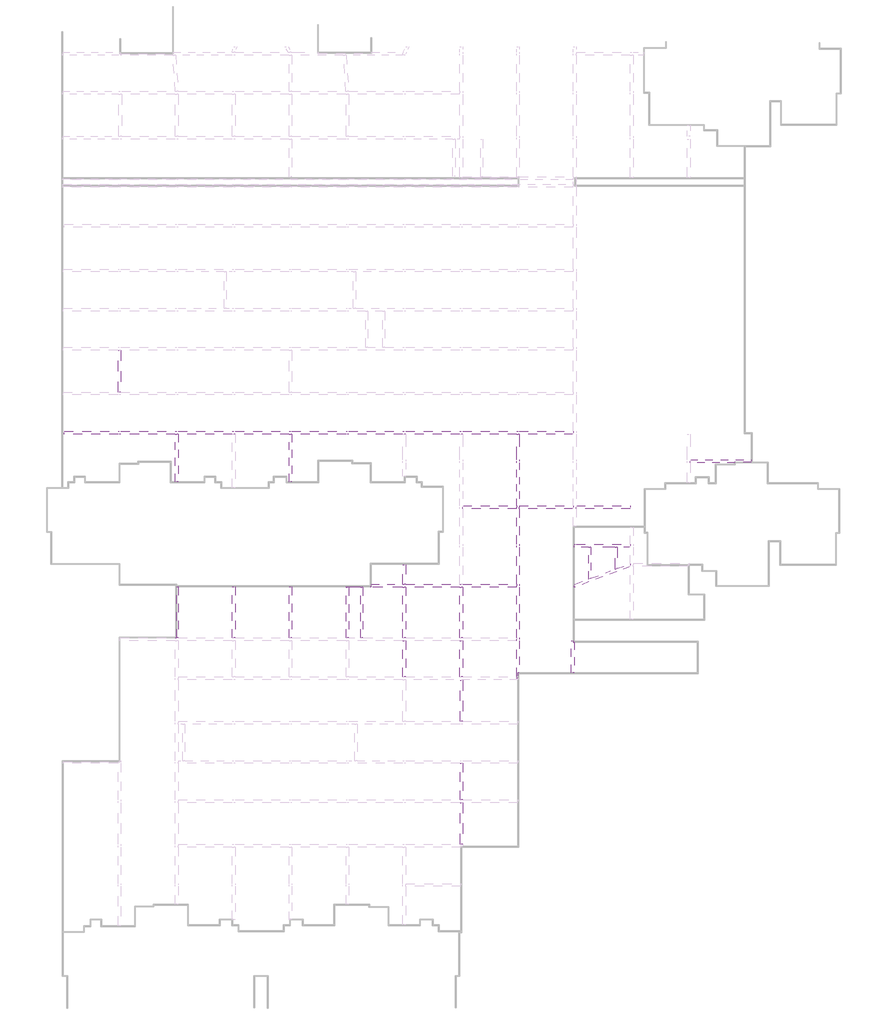
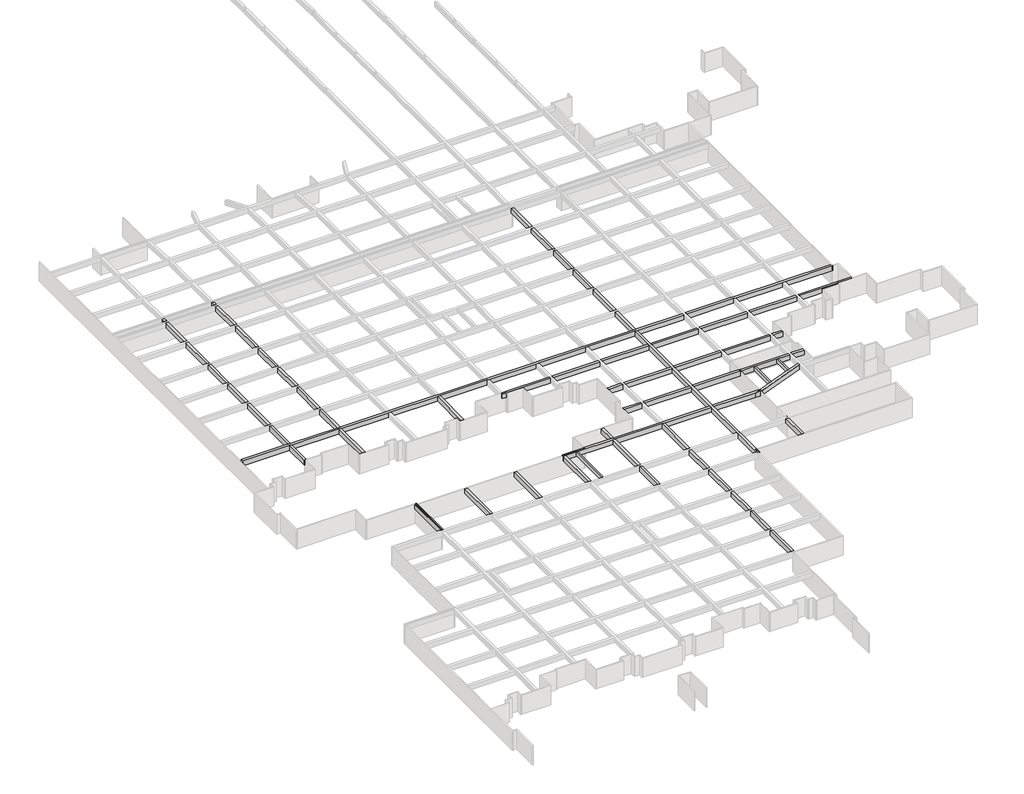
# One storey, part 8 of 14: 28 beams.
"""IFC4 building model written with IfcOpenShell, lengths in millimetres."""

from ifc_helpers import new_model, si_unit, frame, origin, place, context, project, spatial, polyline, outline, extrude, faceted_brep, element, save

model = new_model("IFC4")

# Units and contexts
model_context = context("Model", 3, world=origin())
ifc_project = project(units=[si_unit("LENGTHUNIT", "METRE", prefix="MILLI")], contexts=[model_context])

# Site, building, storey
site = spatial("IfcSite", under=ifc_project)
building = spatial("IfcBuilding", under=site)
storey = spatial("IfcBuildingStorey", under=building, Name="户型图", Elevation=0.0)

# Beams
placement = place(None, origin())
element("IfcBeam", 1, ObjectType="混凝土 - 矩形梁 : KL_beam", at=placement, inside=storey, context=model_context, shape_type="Brep", body=[
    faceted_brep([(-593917.6529954, -163759.4327531, 3300.0), (-593917.6529954, -163759.4327531, 2500.0), (-593917.6529954, -164159.4327531, 2500.0), (-593917.6529954, -164159.4327531, 3300.0), (-522267.6529954, -163759.4327531, 3300.0), (-522267.6529954, -164159.4327531, 3300.0), (-522267.6529954, -164159.4327531, 2500.0), (-522267.6529954, -163759.4327531, 2500.0), (-586331.2602569, -164159.4327531, 3300.0), (-585931.2602569, -164159.4327531, 3300.0), (-578267.6529954, -164159.4327531, 3300.0), (-577867.6529954, -164159.4327531, 3300.0), (-570267.6529954, -164159.4327531, 3300.0), (-569867.6529954, -164159.4327531, 3300.0), (-562267.6529954, -164159.4327531, 3300.0), (-561867.6529954, -164159.4327531, 3300.0), (-554267.6529954, -164159.4327531, 3300.0), (-553867.6529954, -164159.4327531, 3300.0), (-546267.6529954, -164159.4327531, 3300.0), (-545867.6529954, -164159.4327531, 3300.0), (-538267.6529954, -164159.4327531, 3300.0), (-537867.6529954, -164159.4327531, 3300.0), (-530267.6529954, -164159.4327531, 3300.0), (-529867.6529954, -164159.4327531, 3300.0), (-529867.6529954, -163759.4327531, 3300.0), (-530267.6529954, -163759.4327531, 3300.0), (-537867.6529954, -163759.4327531, 3300.0), (-538267.6529954, -163759.4327531, 3300.0), (-545867.6529954, -163759.4327531, 3300.0), (-546267.6529954, -163759.4327531, 3300.0), (-553867.6529954, -163759.4327531, 3300.0), (-554267.6529954, -163759.4327531, 3300.0), (-561867.6529954, -163759.4327531, 3300.0), (-562267.6529954, -163759.4327531, 3300.0), (-569867.6529954, -163759.4327531, 3300.0), (-570267.6529954, -163759.4327531, 3300.0), (-577867.6529954, -163759.4327531, 3300.0), (-578267.6529954, -163759.4327531, 3300.0), (-585931.2602569, -163759.4327531, 3300.0), (-586331.2602569, -163759.4327531, 3300.0), (-586331.2602569, -164159.4327531, 2500.0), (-585931.2602569, -164159.4327531, 2500.0), (-578267.6529954, -164159.4327531, 2500.0), (-577867.6529954, -164159.4327531, 2500.0), (-570267.6529954, -164159.4327531, 2500.0), (-569867.6529954, -164159.4327531, 2500.0), (-562267.6529954, -164159.4327531, 2500.0), (-561867.6529954, -164159.4327531, 2500.0), (-554267.6529954, -164159.4327531, 2500.0), (-553867.6529954, -164159.4327531, 2500.0), (-546267.6529954, -164159.4327531, 2500.0), (-545867.6529954, -164159.4327531, 2500.0), (-538267.6529954, -164159.4327531, 2500.0), (-537867.6529954, -164159.4327531, 2500.0), (-530267.6529954, -164159.4327531, 2500.0), (-529867.6529954, -164159.4327531, 2500.0), (-586331.2602569, -163759.4327531, 2500.0), (-585931.2602569, -163759.4327531, 2500.0), (-578267.6529954, -163759.4327531, 2500.0), (-577867.6529954, -163759.4327531, 2500.0), (-570267.6529954, -163759.4327531, 2500.0), (-569867.6529954, -163759.4327531, 2500.0), (-562267.6529954, -163759.4327531, 2500.0), (-561867.6529954, -163759.4327531, 2500.0), (-554267.6529954, -163759.4327531, 2500.0), (-553867.6529954, -163759.4327531, 2500.0), (-546267.6529954, -163759.4327531, 2500.0), (-545867.6529954, -163759.4327531, 2500.0), (-538267.6529954, -163759.4327531, 2500.0), (-537867.6529954, -163759.4327531, 2500.0), (-530267.6529954, -163759.4327531, 2500.0), (-529867.6529954, -163759.4327531, 2500.0)], [[[0, 1, 2, 3]], [[4, 5, 6, 7]], [[0, 3, 8, 9, 10, 11, 12, 13, 14, 15, 16, 17, 18, 19, 20, 21, 22, 23, 5, 4, 24, 25, 26, 27, 28, 29, 30, 31, 32, 33, 34, 35, 36, 37, 38, 39]], [[3, 2, 40, 41, 42, 43, 44, 45, 46, 47, 48, 49, 50, 51, 52, 53, 54, 55, 6, 5, 23, 22, 21, 20, 19, 18, 17, 16, 15, 14, 13, 12, 11, 10, 9, 8]], [[2, 1, 56, 57, 58, 59, 60, 61, 62, 63, 64, 65, 66, 67, 68, 69, 70, 71, 7, 6, 55, 54, 53, 52, 51, 50, 49, 48, 47, 46, 45, 44, 43, 42, 41, 40]], [[1, 0, 39, 38, 37, 36, 35, 34, 33, 32, 31, 30, 29, 28, 27, 26, 25, 24, 4, 7, 71, 70, 69, 68, 67, 66, 65, 64, 63, 62, 61, 60, 59, 58, 57, 56]]]),
    faceted_brep([(-498227.6529954, -164119.4327531, 3300.0), (-498227.6529954, -163999.4327531, 3300.0), (-498227.6529954, -163759.4327531, 3300.0), (-505867.6529954, -163759.4327531, 3300.0), (-506267.6529954, -163759.4327531, 3300.0), (-513867.6529954, -163759.4327531, 3300.0), (-514267.6529954, -163759.4327531, 3300.0), (-521867.6529954, -163759.4327531, 3300.0), (-521867.6529954, -164159.4327531, 3300.0), (-514267.6529954, -164159.4327531, 3300.0), (-513867.6529954, -164159.4327531, 3300.0), (-506267.6529954, -164159.4327531, 3300.0), (-505867.6529954, -164159.4327531, 3300.0), (-498107.6529954, -164159.4327531, 3300.0), (-498107.6529954, -164119.4327531, 3300.0), (-498107.6529954, -164159.4327531, 2500.0), (-521867.6529954, -164159.4327531, 2500.0), (-514267.6529954, -164159.4327531, 2500.0), (-513867.6529954, -164159.4327531, 2500.0), (-506267.6529954, -164159.4327531, 2500.0), (-505867.6529954, -164159.4327531, 2500.0), (-498227.6529954, -163759.4327531, 2500.0), (-498227.6529954, -164119.4327531, 2500.0), (-498107.6529954, -164119.4327531, 2500.0), (-521867.6529954, -163759.4327531, 2500.0), (-514267.6529954, -163759.4327531, 2500.0), (-513867.6529954, -163759.4327531, 2500.0), (-506267.6529954, -163759.4327531, 2500.0), (-505867.6529954, -163759.4327531, 2500.0)], [[[0, 1, 2, 3, 4, 5, 6, 7, 8, 9, 10, 11, 12, 13, 14]], [[15, 13, 12, 11, 10, 9, 8, 16, 17, 18, 19, 20]], [[21, 22, 23, 15, 20, 19, 18, 17, 16, 24, 25, 26, 27, 28]], [[2, 21, 28, 27, 26, 25, 24, 7, 6, 5, 4, 3]], [[13, 15, 23, 14]], [[0, 22, 21, 2, 1]], [[8, 7, 24, 16]], [[22, 0, 14, 23]]]),
])
element("IfcBeam", 2, ObjectType="混凝土 - 矩形梁 : KL_beam", at=placement, inside=storey, context=model_context, shape_type="Brep", body=[
    faceted_brep([(-586191.2602569, -168257.8565288, 3300.0), (-586071.2602569, -168257.8565288, 3300.0), (-585931.2602569, -168257.8565288, 3300.0), (-585931.2602569, -164159.4327531, 3300.0), (-586331.2602569, -164159.4327531, 3300.0), (-586331.2602569, -168377.8565288, 3300.0), (-586191.2602569, -168377.8565288, 3300.0), (-585931.2602569, -168257.8565288, 2500.0), (-585931.2602569, -164159.4327531, 2500.0), (-586191.2602569, -168257.8565288, 2500.0), (-586191.2602569, -168377.8565288, 2500.0), (-586331.2602569, -168377.8565288, 2500.0), (-586331.2602569, -164159.4327531, 2500.0)], [[[0, 1, 2, 3, 4, 5, 6]], [[2, 7, 8, 3]], [[7, 9, 10, 11, 12, 8]], [[11, 5, 4, 12]], [[5, 11, 10, 6]], [[0, 9, 7, 2, 1]], [[4, 3, 8, 12]], [[9, 0, 6, 10]]]),
    faceted_brep([(-586331.2602569, -128359.4327532, 3300.0), (-585931.2602569, -128359.4327532, 3300.0), (-585931.2602569, -128359.4327532, 2500.0), (-586331.2602569, -128359.4327532, 2500.0), (-585931.2602569, -129034.4327531, 3300.0), (-586331.2602569, -129034.4327531, 3300.0), (-586331.2602569, -129034.4327531, 2500.0), (-585931.2602569, -129034.4327531, 2500.0)], [[[0, 1, 2, 3]], [[4, 5, 6, 7]], [[1, 0, 5, 4]], [[2, 1, 4, 7]], [[3, 2, 7, 6]], [[0, 3, 6, 5]]]),
    faceted_brep([(-586331.2602569, -129434.4327531, 3300.0), (-585931.2602569, -129434.4327531, 3300.0), (-585931.2602569, -129434.4327531, 2500.0), (-586331.2602569, -129434.4327531, 2500.0), (-585931.2602569, -134659.4327531, 3300.0), (-586331.2602569, -134659.4327531, 3300.0), (-586331.2602569, -134659.4327531, 2500.0), (-585931.2602569, -134659.4327531, 2500.0)], [[[0, 1, 2, 3]], [[4, 5, 6, 7]], [[1, 0, 5, 4]], [[2, 1, 4, 7]], [[3, 2, 7, 6]], [[0, 3, 6, 5]]]),
    faceted_brep([(-586331.2602569, -135059.4327531, 3300.0), (-585931.2602569, -135059.4327531, 3300.0), (-585931.2602569, -135059.4327531, 2500.0), (-586331.2602569, -135059.4327531, 2500.0), (-585931.2602569, -140959.4327531, 3300.0), (-586331.2602569, -140959.4327531, 3300.0), (-586331.2602569, -140959.4327531, 2500.0), (-585931.2602569, -140959.4327531, 2500.0)], [[[0, 1, 2, 3]], [[4, 5, 6, 7]], [[1, 0, 5, 4]], [[2, 1, 4, 7]], [[3, 2, 7, 6]], [[0, 3, 6, 5]]]),
    faceted_brep([(-586331.2602569, -141359.4327531, 3300.0), (-585931.2602569, -141359.4327531, 3300.0), (-585931.2602569, -141359.4327531, 2500.0), (-586331.2602569, -141359.4327531, 2500.0), (-585931.2602569, -146459.4327531, 3300.0), (-586331.2602569, -146459.4327531, 3300.0), (-586331.2602569, -146459.4327531, 2500.0), (-585931.2602569, -146459.4327531, 2500.0)], [[[0, 1, 2, 3]], [[4, 5, 6, 7]], [[1, 0, 5, 4]], [[2, 1, 4, 7]], [[3, 2, 7, 6]], [[0, 3, 6, 5]]]),
    faceted_brep([(-586331.2602569, -146859.4327531, 3300.0), (-585931.2602569, -146859.4327531, 3300.0), (-585931.2602569, -146859.4327531, 2500.0), (-586331.2602569, -146859.4327531, 2500.0), (-585931.2602569, -151959.4327531, 3300.0), (-586331.2602569, -151959.4327531, 3300.0), (-586331.2602569, -151959.4327531, 2500.0), (-585931.2602569, -151959.4327531, 2500.0)], [[[0, 1, 2, 3]], [[4, 5, 6, 7]], [[1, 0, 5, 4]], [[2, 1, 4, 7]], [[3, 2, 7, 6]], [[0, 3, 6, 5]]]),
    faceted_brep([(-586331.2602569, -152359.4327531, 3300.0), (-585931.2602569, -152359.4327531, 3300.0), (-585931.2602569, -152359.4327531, 2500.0), (-586331.2602569, -152359.4327531, 2500.0), (-585931.2602569, -158259.4327531, 3300.0), (-586331.2602569, -158259.4327531, 3300.0), (-586331.2602569, -158259.4327531, 2500.0), (-585931.2602569, -158259.4327531, 2500.0)], [[[0, 1, 2, 3]], [[4, 5, 6, 7]], [[1, 0, 5, 4]], [[2, 1, 4, 7]], [[3, 2, 7, 6]], [[0, 3, 6, 5]]]),
    faceted_brep([(-586331.2602569, -158659.4327531, 3300.0), (-585931.2602569, -158659.4327531, 3300.0), (-585931.2602569, -158659.4327531, 2500.0), (-586331.2602569, -158659.4327531, 2500.0), (-585931.2602569, -163759.4327531, 3300.0), (-586331.2602569, -163759.4327531, 3300.0), (-586331.2602569, -163759.4327531, 2500.0), (-585931.2602569, -163759.4327531, 2500.0)], [[[0, 1, 2, 3]], [[4, 5, 6, 7]], [[1, 0, 5, 4]], [[2, 1, 4, 7]], [[3, 2, 7, 6]], [[0, 3, 6, 5]]]),
])
element("IfcBeam", 3, ObjectType="混凝土 - 矩形梁 : KL_beam", at=placement, inside=storey, context=model_context, shape_type="SweptSolid", body=[
    extrude(outline(polyline([(-578267.6529954, -128359.4327532), (-577867.6529954, -128359.4327532), (-577867.6529954, -129034.4327531), (-578267.6529954, -129034.4327531), (-578267.6529954, -128359.4327532)])), frame((0.0, 0.0, 2500.0), z_axis=(0.0, 0.0, 1.0), x_axis=(1.0, 0.0, 0.0)), (0.0, 0.0, 1.0), 800.0),
    extrude(outline(polyline([(-577867.6529954, -170882.8565379), (-578267.6529954, -170882.8565379), (-578267.6529954, -164159.4327531), (-577867.6529954, -164159.4327531), (-577867.6529954, -170882.8565379)])), frame((0.0, 0.0, 2500.0), z_axis=(0.0, 0.0, 1.0), x_axis=(1.0, 0.0, 0.0)), (0.0, 0.0, 1.0), 800.0),
    extrude(outline(polyline([(-578267.6529954, -129434.4327531), (-577867.6529954, -129434.4327531), (-577867.6529954, -134659.4327531), (-578267.6529954, -134659.4327531), (-578267.6529954, -129434.4327531)])), frame((0.0, 0.0, 2500.0), z_axis=(0.0, 0.0, 1.0), x_axis=(1.0, 0.0, 0.0)), (0.0, 0.0, 1.0), 800.0),
    extrude(outline(polyline([(-578267.6529954, -135059.4327531), (-577867.6529954, -135059.4327531), (-577867.6529954, -140959.4327531), (-578267.6529954, -140959.4327531), (-578267.6529954, -135059.4327531)])), frame((0.0, 0.0, 2500.0), z_axis=(0.0, 0.0, 1.0), x_axis=(1.0, 0.0, 0.0)), (0.0, 0.0, 1.0), 800.0),
    extrude(outline(polyline([(-578267.6529954, -141359.4327531), (-577867.6529954, -141359.4327531), (-577867.6529954, -146459.4327531), (-578267.6529954, -146459.4327531), (-578267.6529954, -141359.4327531)])), frame((0.0, 0.0, 2500.0), z_axis=(0.0, 0.0, 1.0), x_axis=(1.0, 0.0, 0.0)), (0.0, 0.0, 1.0), 800.0),
    extrude(outline(polyline([(-578267.6529954, -146859.4327531), (-577867.6529954, -146859.4327531), (-577867.6529954, -151959.4327531), (-578267.6529954, -151959.4327531), (-578267.6529954, -146859.4327531)])), frame((0.0, 0.0, 2500.0), z_axis=(0.0, 0.0, 1.0), x_axis=(1.0, 0.0, 0.0)), (0.0, 0.0, 1.0), 800.0),
    extrude(outline(polyline([(-578267.6529954, -152359.4327531), (-577867.6529954, -152359.4327531), (-577867.6529954, -158259.4327531), (-578267.6529954, -158259.4327531), (-578267.6529954, -152359.4327531)])), frame((0.0, 0.0, 2500.0), z_axis=(0.0, 0.0, 1.0), x_axis=(1.0, 0.0, 0.0)), (0.0, 0.0, 1.0), 800.0),
    extrude(outline(polyline([(-578267.6529954, -158659.4327531), (-577867.6529954, -158659.4327531), (-577867.6529954, -163759.4327531), (-578267.6529954, -163759.4327531), (-578267.6529954, -158659.4327531)])), frame((0.0, 0.0, 2500.0), z_axis=(0.0, 0.0, 1.0), x_axis=(1.0, 0.0, 0.0)), (0.0, 0.0, 1.0), 800.0),
])
element("IfcBeam", 4, ObjectType="混凝土 - 矩形梁 : KL_beam", at=placement, inside=storey, context=model_context, shape_type="Brep", body=[
    faceted_brep([(-529867.6529954, -198534.4327531, 2500.0), (-529867.6529954, -198534.4327531, 3300.0), (-529997.7352575, -198534.4327531, 3300.0), (-529997.7352575, -198534.4327531, 2500.0), (-529867.6529954, -197850.9174567, 3300.0), (-529997.7352575, -197850.9174567, 3300.0), (-529867.6529954, -197850.9174567, 2500.0), (-529997.7352575, -197850.9174567, 2500.0)], [[[0, 1, 2, 3]], [[2, 1, 4, 5]], [[1, 0, 6, 4]], [[3, 2, 5, 7]], [[5, 4, 6, 7]], [[0, 3, 7, 6]]]),
    faceted_brep([(-530267.6529954, -198534.4327531, 2500.0), (-530267.6529954, -198534.4327531, 3300.0), (-530267.6529954, -198334.4327531, 3300.0), (-530267.6529954, -193242.8565135, 3300.0), (-530267.6529954, -192842.8565135, 3300.0), (-530267.6529954, -185692.8565135, 3300.0), (-530267.6529954, -185292.8565135, 3300.0), (-530267.6529954, -180052.8565433, 3300.0), (-530267.6529954, -179652.8565433, 3300.0), (-530267.6529954, -174657.5200046, 3300.0), (-530267.6529954, -174257.5200046, 3300.0), (-530267.6529954, -168200.507479, 3300.0), (-530267.6529954, -167800.507479, 3300.0), (-530267.6529954, -164159.4327531, 3300.0), (-530267.6529954, -164159.4327531, 2500.0), (-530267.6529954, -167800.507479, 2500.0), (-530267.6529954, -168200.507479, 2500.0), (-530267.6529954, -174257.5200046, 2500.0), (-530267.6529954, -174657.5200046, 2500.0), (-530267.6529954, -179652.8565433, 2500.0), (-530267.6529954, -180052.8565433, 2500.0), (-530267.6529954, -185292.8565135, 2500.0), (-530267.6529954, -185692.8565135, 2500.0), (-530267.6529954, -192842.8565135, 2500.0), (-530267.6529954, -193242.8565135, 2500.0), (-530267.6529954, -198334.4327531, 2500.0), (-529867.6529954, -164159.4327531, 2500.0), (-529867.6529954, -167800.507479, 2500.0), (-529867.6529954, -168200.507479, 2500.0), (-529867.6529954, -174257.5200046, 2500.0), (-529867.6529954, -174657.5200046, 2500.0), (-529867.6529954, -179652.8565433, 2500.0), (-529867.6529954, -180052.8565433, 2500.0), (-529867.6529954, -185292.8565135, 2500.0), (-529867.6529954, -185692.8565135, 2500.0), (-529867.6529954, -192842.8565135, 2500.0), (-529867.6529954, -193242.8565135, 2500.0), (-529867.6529954, -197730.9174567, 2500.0), (-530117.7352575, -197730.9174567, 2500.0), (-530117.7352575, -198534.4327531, 2500.0), (-529867.6529954, -164159.4327531, 3300.0), (-530117.7352575, -197730.9174567, 3300.0), (-530117.7352575, -198534.4327531, 3300.0), (-529867.6529954, -197730.9174567, 3300.0), (-529997.7352575, -197730.9174567, 3300.0), (-529867.6529954, -193242.8565135, 3300.0), (-529867.6529954, -192842.8565135, 3300.0), (-529867.6529954, -185692.8565135, 3300.0), (-529867.6529954, -185292.8565135, 3300.0), (-529867.6529954, -180052.8565433, 3300.0), (-529867.6529954, -179652.8565433, 3300.0), (-529867.6529954, -174657.5200046, 3300.0), (-529867.6529954, -174257.5200046, 3300.0), (-529867.6529954, -168200.507479, 3300.0), (-529867.6529954, -167800.507479, 3300.0)], [[[0, 1, 2, 3, 4, 5, 6, 7, 8, 9, 10, 11, 12, 13, 14, 15, 16, 17, 18, 19, 20, 21, 22, 23, 24, 25]], [[0, 25, 24, 23, 22, 21, 20, 19, 18, 17, 16, 15, 14, 26, 27, 28, 29, 30, 31, 32, 33, 34, 35, 36, 37, 38, 39]], [[13, 40, 26, 14]], [[38, 41, 42, 39]], [[41, 38, 37, 43, 44]], [[1, 0, 39, 42]], [[13, 12, 11, 10, 9, 8, 7, 6, 5, 4, 3, 2, 1, 42, 41, 44, 43, 45, 46, 47, 48, 49, 50, 51, 52, 53, 54, 40]], [[26, 40, 54, 53, 52, 51, 50, 49, 48, 47, 46, 45, 43, 37, 36, 35, 34, 33, 32, 31, 30, 29, 28, 27]]]),
    faceted_brep([(-530267.6529954, -129434.4327531, 3300.0), (-529867.6529954, -129434.4327531, 3300.0), (-529867.6529954, -129434.4327531, 2500.0), (-530267.6529954, -129434.4327531, 2500.0), (-529867.6529954, -134659.4327531, 3300.0), (-530267.6529954, -134659.4327531, 3300.0), (-530267.6529954, -134659.4327531, 2500.0), (-529867.6529954, -134659.4327531, 2500.0)], [[[0, 1, 2, 3]], [[4, 5, 6, 7]], [[1, 0, 5, 4]], [[0, 3, 6, 5]], [[3, 2, 7, 6]], [[2, 1, 4, 7]]]),
    faceted_brep([(-530267.6529954, -135059.4327531, 3300.0), (-529867.6529954, -135059.4327531, 3300.0), (-529867.6529954, -135059.4327531, 2500.0), (-530267.6529954, -135059.4327531, 2500.0), (-529867.6529954, -140959.4327531, 3300.0), (-530267.6529954, -140959.4327531, 3300.0), (-530267.6529954, -140959.4327531, 2500.0), (-529867.6529954, -140959.4327531, 2500.0)], [[[0, 1, 2, 3]], [[4, 5, 6, 7]], [[1, 0, 5, 4]], [[0, 3, 6, 5]], [[3, 2, 7, 6]], [[2, 1, 4, 7]]]),
    faceted_brep([(-530267.6529954, -141359.4327531, 3300.0), (-529867.6529954, -141359.4327531, 3300.0), (-529867.6529954, -141359.4327531, 2500.0), (-530267.6529954, -141359.4327531, 2500.0), (-529867.6529954, -146459.4327531, 3300.0), (-530267.6529954, -146459.4327531, 3300.0), (-530267.6529954, -146459.4327531, 2500.0), (-529867.6529954, -146459.4327531, 2500.0)], [[[0, 1, 2, 3]], [[4, 5, 6, 7]], [[1, 0, 5, 4]], [[0, 3, 6, 5]], [[3, 2, 7, 6]], [[2, 1, 4, 7]]]),
    faceted_brep([(-530267.6529954, -146859.4327531, 3300.0), (-529867.6529954, -146859.4327531, 3300.0), (-529867.6529954, -146859.4327531, 2500.0), (-530267.6529954, -146859.4327531, 2500.0), (-529867.6529954, -151959.4327531, 3300.0), (-530267.6529954, -151959.4327531, 3300.0), (-530267.6529954, -151959.4327531, 2500.0), (-529867.6529954, -151959.4327531, 2500.0)], [[[0, 1, 2, 3]], [[4, 5, 6, 7]], [[1, 0, 5, 4]], [[0, 3, 6, 5]], [[3, 2, 7, 6]], [[2, 1, 4, 7]]]),
    faceted_brep([(-530267.6529954, -152359.4327531, 3300.0), (-529867.6529954, -152359.4327531, 3300.0), (-529867.6529954, -152359.4327531, 2500.0), (-530267.6529954, -152359.4327531, 2500.0), (-529867.6529954, -158259.4327531, 3300.0), (-530267.6529954, -158259.4327531, 3300.0), (-530267.6529954, -158259.4327531, 2500.0), (-529867.6529954, -158259.4327531, 2500.0)], [[[0, 1, 2, 3]], [[4, 5, 6, 7]], [[1, 0, 5, 4]], [[0, 3, 6, 5]], [[3, 2, 7, 6]], [[2, 1, 4, 7]]]),
    faceted_brep([(-530267.6529954, -158659.4327531, 3300.0), (-529867.6529954, -158659.4327531, 3300.0), (-529867.6529954, -158659.4327531, 2500.0), (-530267.6529954, -158659.4327531, 2500.0), (-529867.6529954, -163759.4327531, 3300.0), (-530267.6529954, -163759.4327531, 3300.0), (-530267.6529954, -163759.4327531, 2500.0), (-529867.6529954, -163759.4327531, 2500.0)], [[[0, 1, 2, 3]], [[4, 5, 6, 7]], [[1, 0, 5, 4]], [[0, 3, 6, 5]], [[3, 2, 7, 6]], [[2, 1, 4, 7]]]),
])
element("IfcBeam", 5, ObjectType="混凝土 - 矩形梁 : KL_beam", at=placement, inside=storey, context=model_context, shape_type="Brep", body=[
    faceted_brep([(-554067.6529954, -168200.507479, 2500.0), (-554067.6529954, -168200.507479, 3300.0), (-554067.6529954, -167952.8565288, 3300.0), (-554067.6529954, -167952.8565288, 2500.0), (-553441.260255, -168200.507479, 3300.0), (-553441.260255, -167952.8565288, 3300.0), (-553441.260255, -168200.507479, 2500.0), (-553441.260255, -167952.8565288, 2500.0)], [[[0, 1, 2, 3]], [[2, 1, 4, 5]], [[1, 0, 6, 4]], [[3, 2, 5, 7]], [[5, 4, 6, 7]], [[0, 3, 7, 6]]]),
    faceted_brep([(-522267.6529954, -167800.507479, 3300.0), (-522267.6529954, -167800.507479, 2500.0), (-529867.6529954, -167800.507479, 2500.0), (-529867.6529954, -167800.507479, 3300.0), (-522267.6529954, -168200.507479, 2500.0), (-529867.6529954, -168200.507479, 2500.0), (-522267.6529954, -168200.507479, 3300.0), (-529867.6529954, -168200.507479, 3300.0)], [[[0, 1, 2, 3]], [[1, 4, 5, 2]], [[0, 6, 4, 1]], [[3, 2, 5, 7]], [[6, 0, 3, 7]], [[4, 6, 7, 5]]]),
    faceted_brep([(-497277.6529954, -167800.507479, 3300.0), (-497277.6529954, -168097.2169847, 3300.0), (-497277.6529954, -168097.2169847, 2500.0), (-497277.6529954, -167800.507479, 2500.0), (-505867.6529954, -168200.507479, 3300.0), (-505867.6529954, -167800.507479, 3300.0), (-505867.6529954, -167800.507479, 2500.0), (-505867.6529954, -168200.507479, 2500.0), (-499624.2878989, -168200.507479, 3300.0), (-499624.2878989, -168097.2169847, 3300.0), (-499504.2878989, -168097.2169847, 3300.0), (-499624.2878989, -168097.2169847, 2500.0), (-499624.2878989, -168200.507479, 2500.0)], [[[0, 1, 2, 3]], [[4, 5, 6, 7]], [[1, 0, 5, 4, 8, 9, 10]], [[0, 3, 6, 5]], [[3, 2, 11, 12, 7, 6]], [[4, 7, 12, 8]], [[2, 1, 10, 9, 11]], [[11, 9, 8, 12]]]),
    faceted_brep([(-521867.6529954, -168200.507479, 3300.0), (-521867.6529954, -167800.507479, 3300.0), (-521867.6529954, -167800.507479, 2500.0), (-521867.6529954, -168200.507479, 2500.0), (-514267.6529954, -168200.507479, 3300.0), (-514267.6529954, -167800.507479, 3300.0), (-514267.6529954, -167800.507479, 2500.0), (-514267.6529954, -168200.507479, 2500.0)], [[[0, 1, 2, 3]], [[1, 0, 4, 5]], [[2, 1, 5, 6]], [[3, 2, 6, 7]], [[0, 3, 7, 4]], [[5, 4, 7, 6]]]),
    faceted_brep([(-553867.6529954, -167800.507479, 3300.0), (-553867.6529954, -167800.507479, 2500.0), (-553867.6529954, -167832.8565288, 2500.0), (-553867.6529954, -167832.8565288, 3300.0), (-546267.6529954, -167800.507479, 3300.0), (-546267.6529954, -168200.507479, 3300.0), (-546267.6529954, -168200.507479, 2500.0), (-546267.6529954, -167800.507479, 2500.0), (-553321.260255, -168200.507479, 2500.0), (-553321.260255, -167832.8565288, 2500.0), (-553321.260255, -167832.8565288, 3300.0), (-553321.260255, -168200.507479, 3300.0), (-553321.260255, -167952.8565288, 3300.0)], [[[0, 1, 2, 3]], [[4, 5, 6, 7]], [[1, 0, 4, 7]], [[1, 7, 6, 8, 9, 2]], [[9, 10, 3, 2]], [[10, 9, 8, 11, 12]], [[4, 0, 3, 10, 12, 11, 5]], [[6, 5, 11, 8]]]),
    faceted_brep([(-545867.6529954, -168200.507479, 3300.0), (-545867.6529954, -167800.507479, 3300.0), (-545867.6529954, -167800.507479, 2500.0), (-545867.6529954, -168200.507479, 2500.0), (-538267.6529954, -168200.507479, 3300.0), (-538267.6529954, -167800.507479, 3300.0), (-538267.6529954, -168200.507479, 2500.0), (-538267.6529954, -167800.507479, 2500.0)], [[[0, 1, 2, 3]], [[1, 0, 4, 5]], [[0, 3, 6, 4]], [[7, 5, 4, 6]], [[2, 1, 5, 7]], [[3, 2, 7, 6]]]),
    faceted_brep([(-537867.6529954, -167800.507479, 3300.0), (-537867.6529954, -167800.507479, 2500.0), (-537867.6529954, -168200.507479, 2500.0), (-537867.6529954, -168200.507479, 3300.0), (-530267.6529954, -168200.507479, 3300.0), (-530267.6529954, -167800.507479, 3300.0), (-530267.6529954, -168200.507479, 2500.0), (-530267.6529954, -167800.507479, 2500.0)], [[[0, 1, 2, 3]], [[0, 3, 4, 5]], [[3, 2, 6, 4]], [[7, 5, 4, 6]], [[1, 0, 5, 7]], [[2, 1, 7, 6]]]),
    faceted_brep([(-513867.6529954, -168200.507479, 3300.0), (-513867.6529954, -167800.507479, 3300.0), (-513867.6529954, -167800.507479, 2500.0), (-513867.6529954, -168200.507479, 2500.0), (-506267.6529954, -168200.507479, 3300.0), (-506267.6529954, -167800.507479, 3300.0), (-506267.6529954, -167800.507479, 2500.0), (-506267.6529954, -168200.507479, 2500.0)], [[[0, 1, 2, 3]], [[1, 0, 4, 5]], [[2, 1, 5, 6]], [[3, 2, 6, 7]], [[0, 3, 7, 4]], [[5, 4, 7, 6]]]),
])
element("IfcBeam", 6, ObjectType="混凝土 - 矩形梁 : KL_beam", at=placement, inside=storey, context=model_context, shape_type="SweptSolid", body=[
    extrude(outline(polyline([(-561867.6529954, -170882.8565379), (-562267.6529954, -170882.8565379), (-562267.6529954, -164159.4327531), (-561867.6529954, -164159.4327531), (-561867.6529954, -170882.8565379)])), frame((0.0, 0.0, 2500.0), z_axis=(0.0, 0.0, 1.0), x_axis=(1.0, 0.0, 0.0)), (0.0, 0.0, 1.0), 800.0),
])
element("IfcBeam", 7, ObjectType="混凝土 - 矩形梁 : KL_beam", at=placement, inside=storey, context=model_context, shape_type="SweptSolid", body=[
    extrude(outline(polyline([(-522267.6529954, -174257.5200046), (-522267.6529954, -174657.5200046), (-529867.6529954, -174657.5200046), (-529867.6529954, -174257.5200046), (-522267.6529954, -174257.5200046)])), frame((0.0, 0.0, 2500.0), z_axis=(0.0, 0.0, 1.0), x_axis=(1.0, 0.0, 0.0)), (0.0, 0.0, 1.0), 800.0),
])
element("IfcBeam", 8, ObjectType="混凝土 - 矩形梁 : KL_beam", at=placement, inside=storey, context=model_context, shape_type="SweptSolid", body=[
    extrude(outline(polyline([(-521867.6529954, -174657.5200046), (-521867.6529954, -174257.5200046), (-514267.6529954, -174257.5200046), (-514267.6529954, -174657.5200046), (-521867.6529954, -174657.5200046)])), frame((0.0, 0.0, 2500.0), z_axis=(0.0, 0.0, 1.0), x_axis=(1.0, 0.0, 0.0)), (0.0, 0.0, 1.0), 800.0),
    extrude(outline(polyline([(-512303.9222774, -174257.5200046), (-512303.9222774, -174657.5200046), (-513867.6529954, -174657.5200046), (-513867.6529954, -174257.5200046), (-512303.9222774, -174257.5200046)])), frame((0.0, 0.0, 2500.0), z_axis=(0.0, 0.0, 1.0), x_axis=(1.0, 0.0, 0.0)), (0.0, 0.0, 1.0), 800.0),
])
element("IfcBeam", 9, ObjectType="混凝土 - 矩形梁 : KL_beam", at=placement, inside=storey, context=model_context, shape_type="SweptSolid", body=[
    extrude(outline(polyline([(-530267.6529954, -174257.5200046), (-530267.6529954, -174657.5200046), (-537867.6529954, -174657.5200046), (-537867.6529954, -174257.5200046), (-530267.6529954, -174257.5200046)])), frame((0.0, 0.0, 2500.0), z_axis=(0.0, 0.0, 1.0), x_axis=(1.0, 0.0, 0.0)), (0.0, 0.0, 1.0), 800.0),
    extrude(outline(polyline([(-540571.2602521, -174657.5200046), (-540571.2602521, -174257.5200046), (-538267.6529954, -174257.5200046), (-538267.6529954, -174657.5200046), (-540571.2602521, -174657.5200046)])), frame((0.0, 0.0, 2500.0), z_axis=(0.0, 0.0, 1.0), x_axis=(1.0, 0.0, 0.0)), (0.0, 0.0, 1.0), 800.0),
])
element("IfcBeam", 10, ObjectType="混凝土 - 矩形梁 : KL_beam", at=placement, inside=storey, context=model_context, shape_type="Brep", body=[
    faceted_brep([(-511864.0912647, -179652.8565433, 3300.0), (-511864.0912647, -180052.8565433, 3300.0), (-511864.0912647, -180052.8565433, 2500.0), (-511864.0912647, -179652.8565433, 2500.0), (-513867.6529954, -179652.8565433, 3300.0), (-513867.6529954, -180052.8565433, 3300.0), (-513867.6529954, -180052.8565433, 2500.0), (-513867.6529954, -179652.8565433, 2500.0)], [[[0, 1, 2, 3]], [[1, 0, 4, 5]], [[2, 1, 5, 6]], [[3, 2, 6, 7]], [[0, 3, 7, 4]], [[5, 4, 7, 6]]]),
    faceted_brep([(-541171.2602521, -180052.8565433, 3300.0), (-541171.2602521, -179652.8565433, 3300.0), (-541171.2602521, -179652.8565433, 2500.0), (-541171.2602521, -180052.8565433, 2500.0), (-538267.6529954, -179652.8565433, 3300.0), (-538267.6529954, -180052.8565433, 3300.0), (-538267.6529954, -180052.8565433, 2500.0), (-538267.6529954, -179652.8565433, 2500.0)], [[[0, 1, 2, 3]], [[4, 5, 6, 7]], [[1, 0, 5, 4]], [[0, 3, 6, 5]], [[3, 2, 7, 6]], [[2, 1, 4, 7]]]),
    faceted_brep([(-537867.6529954, -180052.8565433, 3300.0), (-537867.6529954, -179652.8565433, 3300.0), (-537867.6529954, -179652.8565433, 2500.0), (-537867.6529954, -180052.8565433, 2500.0), (-530267.6529954, -179652.8565433, 3300.0), (-530267.6529954, -180052.8565433, 3300.0), (-530267.6529954, -180052.8565433, 2500.0), (-530267.6529954, -179652.8565433, 2500.0)], [[[0, 1, 2, 3]], [[4, 5, 6, 7]], [[1, 0, 5, 4]], [[0, 3, 6, 5]], [[3, 2, 7, 6]], [[2, 1, 4, 7]]]),
    faceted_brep([(-529867.6529954, -180052.8565433, 3300.0), (-529867.6529954, -179652.8565433, 3300.0), (-529867.6529954, -179652.8565433, 2500.0), (-529867.6529954, -180052.8565433, 2500.0), (-522303.9222774, -179652.8565433, 3300.0), (-522303.9222774, -180052.8565433, 3300.0), (-522303.9222774, -180052.8565433, 2500.0), (-522303.9222774, -179652.8565433, 2500.0)], [[[0, 1, 2, 3]], [[4, 5, 6, 7]], [[1, 0, 5, 4]], [[0, 3, 6, 5]], [[3, 2, 7, 6]], [[2, 1, 4, 7]]]),
    faceted_brep([(-514267.6529954, -179652.8565433, 3300.0), (-514267.6529954, -180052.8565433, 3300.0), (-514267.6529954, -180052.8565433, 2500.0), (-514267.6529954, -179652.8565433, 2500.0), (-521867.6529954, -179652.8565433, 3300.0), (-522183.9222774, -179652.8565433, 3300.0), (-522183.9222774, -180052.8565433, 3300.0), (-520117.6529954, -180052.8565433, 3300.0), (-519817.6529954, -180052.8565433, 3300.0), (-516417.6683344, -180052.8565433, 3300.0), (-516117.6683344, -180052.8565433, 3300.0), (-522183.9222774, -180052.8565433, 2500.0), (-522183.9222774, -179652.8565433, 2500.0), (-521867.6529954, -179652.8565433, 2500.0)], [[[0, 1, 2, 3]], [[1, 0, 4, 5, 6, 7, 8, 9, 10]], [[2, 1, 10, 9, 8, 7, 6, 11]], [[3, 2, 11, 12, 13]], [[0, 3, 13, 12, 5, 4]], [[6, 5, 12, 11]]]),
])
element("IfcBeam", 11, ObjectType="混凝土 - 矩形梁 : KL_beam", at=placement, inside=storey, context=model_context, shape_type="Brep", body=[
    faceted_brep([(-523181.5016488, -185692.8565135, 3300.0), (-522303.9222774, -185692.8565135, 3300.0), (-522303.9222774, -185367.2051019, 3300.0), (-523181.5016488, -185692.8565135, 2500.0), (-522303.9222774, -185367.2051019, 2500.0), (-522303.9222774, -185692.8565135, 2500.0)], [[[0, 1, 2]], [[3, 0, 2, 4]], [[5, 3, 4]], [[2, 1, 5, 4]], [[0, 3, 5, 1]]]),
    faceted_brep([(-514267.6529954, -182811.7651217, 2500.0), (-514267.6529954, -182811.7651217, 3300.0), (-522031.7414738, -185692.8565135, 3300.0), (-522031.7414738, -185692.8565135, 2500.0), (-514267.6529954, -182385.1130875, 3300.0), (-514267.6529954, -182385.1130875, 2500.0), (-522183.9222774, -185692.8565135, 3300.0), (-522183.9222774, -185692.8565135, 2500.0), (-522183.9222774, -185322.6756033, 3300.0), (-522183.9222774, -185322.6756033, 2500.0), (-516117.6683344, -183071.6152162, 3300.0), (-516417.6683344, -183182.9389627, 3300.0), (-519817.6529954, -184444.6023977, 3300.0), (-520117.6529954, -184555.9261442, 3300.0), (-522103.564517, -185292.8565135, 3300.0), (-522103.564517, -185292.8565135, 2500.0)], [[[0, 1, 2, 3]], [[4, 1, 0, 5]], [[3, 2, 6, 7]], [[6, 8, 9, 7]], [[1, 4, 10, 11, 12, 13, 14, 8, 6, 2]], [[4, 5, 15, 9, 8, 14, 13, 12, 11, 10]], [[5, 0, 3, 7, 9, 15]]]),
])
element("IfcBeam", 12, ObjectType="混凝土 - 矩形梁 : KL_beam", at=placement, inside=storey, context=model_context, shape_type="Brep", body=[
    faceted_brep([(-550841.260255, -185292.8565135, 3300.0), (-554267.6529954, -185292.8565135, 3300.0), (-554267.6529954, -185532.8564588, 3300.0), (-550841.260255, -185532.8564588, 3300.0), (-550841.260255, -185292.8565135, 2500.0), (-554267.6529954, -185292.8565135, 2500.0), (-550841.260255, -185532.8564588, 2500.0), (-554267.6529954, -185532.8564588, 2500.0)], [[[0, 1, 2, 3]], [[0, 4, 5, 1]], [[5, 4, 6, 7]], [[4, 0, 3, 6]], [[3, 2, 7, 6]], [[1, 5, 7, 2]]]),
    faceted_brep([(-530267.6529954, -185692.8565135, 2500.0), (-530267.6529954, -185692.8565135, 3300.0), (-537867.6529954, -185692.8565135, 3300.0), (-538267.6529954, -185692.8565135, 3300.0), (-545867.6529954, -185692.8565135, 3300.0), (-546267.6529954, -185692.8565135, 3300.0), (-551917.6529953, -185692.8565135, 3300.0), (-552217.6529953, -185692.8565135, 3300.0), (-553867.6529954, -185692.8565135, 3300.0), (-554267.6529954, -185692.8565135, 3300.0), (-554267.6529954, -185692.8565135, 2500.0), (-553867.6529954, -185692.8565135, 2500.0), (-546267.6529954, -185692.8565135, 2500.0), (-545867.6529954, -185692.8565135, 2500.0), (-538267.6529954, -185692.8565135, 2500.0), (-537867.6529954, -185692.8565135, 2500.0), (-530267.6529954, -185292.8565135, 3300.0), (-530267.6529954, -185292.8565135, 2500.0), (-550721.260255, -185652.8564588, 2500.0), (-550721.260255, -185652.8564588, 3300.0), (-550721.260255, -185292.8565135, 3300.0), (-550721.260255, -185292.8565135, 2500.0), (-554267.6529954, -185652.8564588, 2500.0), (-554267.6529954, -185652.8564588, 3300.0), (-550841.260255, -185652.8564588, 3300.0), (-537867.6529954, -185292.8565135, 2500.0), (-538267.6529954, -185292.8565135, 2500.0), (-545867.6529954, -185292.8565135, 2500.0), (-546267.6529954, -185292.8565135, 2500.0), (-546267.6529954, -185292.8565135, 3300.0), (-545867.6529954, -185292.8565135, 3300.0), (-538267.6529954, -185292.8565135, 3300.0), (-537867.6529954, -185292.8565135, 3300.0)], [[[0, 1, 2, 3, 4, 5, 6, 7, 8, 9, 10, 11, 12, 13, 14, 15]], [[16, 1, 0, 17]], [[18, 19, 20, 21]], [[19, 18, 22, 23, 24]], [[16, 17, 25, 26, 27, 28, 21, 20, 29, 30, 31, 32]], [[1, 16, 32, 31, 30, 29, 20, 19, 24, 23, 9, 8, 7, 6, 5, 4, 3, 2]], [[17, 0, 15, 14, 13, 12, 11, 10, 22, 18, 21, 28, 27, 26, 25]], [[10, 9, 23, 22]]]),
    faceted_brep([(-523181.5016488, -185692.8565135, 3300.0), (-523181.5016488, -185692.8565135, 2500.0), (-522303.9222774, -185367.2051019, 2500.0), (-522303.9222774, -185367.2051019, 3300.0), (-529867.6529954, -185692.8565135, 3300.0), (-529867.6529954, -185292.8565135, 3300.0), (-529867.6529954, -185292.8565135, 2500.0), (-529867.6529954, -185692.8565135, 2500.0), (-522303.9222774, -185292.8565135, 3300.0), (-522303.9222774, -185292.8565135, 2500.0)], [[[0, 1, 2, 3]], [[4, 5, 6, 7]], [[5, 4, 0, 3, 8]], [[6, 5, 8, 9]], [[7, 6, 9, 2, 1]], [[1, 0, 4, 7]], [[3, 2, 9, 8]]]),
    faceted_brep([(-522183.9222774, -185322.6756033, 2500.0), (-522183.9222774, -185322.6756033, 3300.0), (-522183.9222774, -185292.8565135, 3300.0), (-522183.9222774, -185292.8565135, 2500.0), (-522103.564517, -185292.8565135, 2500.0), (-522103.564517, -185292.8565135, 3300.0)], [[[0, 1, 2, 3]], [[4, 5, 1, 0]], [[1, 5, 2]], [[5, 4, 3, 2]], [[4, 0, 3]]]),
])
element("IfcBeam", 13, ObjectType="混凝土 - 矩形梁 : KL_beam", at=placement, inside=storey, context=model_context, shape_type="SweptSolid", body=[
    extrude(outline(polyline([(-546267.6529954, -182524.5398935), (-545867.6529954, -182524.5398935), (-545867.6529954, -185292.8565135), (-546267.6529954, -185292.8565135), (-546267.6529954, -182524.5398935)])), frame((0.0, 0.0, 2500.0), z_axis=(0.0, 0.0, 1.0), x_axis=(1.0, 0.0, 0.0)), (0.0, 0.0, 1.0), 800.0),
])
element("IfcBeam", 14, ObjectType="混凝土 - 矩形梁 : KL_beam", at=placement, inside=storey, context=model_context, shape_type="Brep", body=[
    faceted_brep([(-577867.6529954, -185371.5491398, 3300.0), (-577867.6529954, -185371.5491398, 2500.0), (-578071.2602569, -185371.5491398, 2500.0), (-578071.2602569, -185371.5491398, 3300.0), (-577867.6529954, -185532.8564588, 3300.0), (-577867.6529954, -185532.8564588, 2500.0), (-578071.2602569, -185532.8564588, 2500.0), (-578071.2602569, -185532.8564588, 3300.0), (-578071.2602569, -185431.2417661, 3300.0)], [[[0, 1, 2, 3]], [[1, 0, 4, 5]], [[2, 1, 5, 6]], [[5, 4, 7, 6]], [[3, 2, 6, 7, 8]], [[0, 3, 8, 7, 4]]]),
    faceted_brep([(-578191.2602569, -185431.2417661, 3300.0), (-578267.6529954, -185431.2417661, 3300.0), (-578267.6529954, -192711.2417661, 3300.0), (-578191.2602569, -192711.2417661, 3300.0), (-578267.6529954, -185431.2417661, 2500.0), (-578191.2602569, -185431.2417661, 2500.0), (-578191.2602569, -192711.2417661, 2500.0), (-578267.6529954, -192711.2417661, 2500.0)], [[[0, 1, 2, 3]], [[4, 1, 0, 5]], [[5, 0, 3, 6]], [[3, 2, 7, 6]], [[4, 5, 6, 7]], [[1, 4, 7, 2]]]),
    faceted_brep([(-578267.6529954, -192842.8565135, 2500.0), (-578267.6529954, -192842.8565135, 3300.0), (-578267.6529954, -192831.2417661, 3300.0), (-578267.6529954, -192831.2417661, 2500.0), (-577867.6529954, -192842.8565135, 3300.0), (-577867.6529954, -192842.8565135, 2500.0), (-578071.2602569, -192831.2417661, 2500.0), (-578071.2602569, -192831.2417661, 3300.0), (-578071.2602569, -185652.8564588, 3300.0), (-578071.2602569, -185652.8564588, 2500.0), (-578191.2602569, -192831.2417661, 3300.0), (-577867.6529954, -185652.8564588, 3300.0), (-577867.6529954, -185652.8564588, 2500.0)], [[[0, 1, 2, 3]], [[4, 1, 0, 5]], [[6, 7, 8, 9]], [[7, 6, 3, 2, 10]], [[1, 4, 11, 8, 7, 10, 2]], [[11, 12, 9, 8]], [[4, 5, 12, 11]], [[5, 0, 3, 6, 9, 12]]]),
])
element("IfcBeam", 15, ObjectType="混凝土 - 矩形梁 : KL_beam", at=placement, inside=storey, context=model_context, shape_type="SweptSolid", body=[
    extrude(outline(polyline([(-570267.6529954, -185652.8564588), (-569867.6529954, -185652.8564588), (-569867.6529954, -192842.8565135), (-570267.6529954, -192842.8565135), (-570267.6529954, -185652.8564588)])), frame((0.0, 0.0, 2500.0), z_axis=(0.0, 0.0, 1.0), x_axis=(1.0, 0.0, 0.0)), (0.0, 0.0, 1.0), 800.0),
])
element("IfcBeam", 16, ObjectType="混凝土 - 矩形梁 : KL_beam", at=placement, inside=storey, context=model_context, shape_type="SweptSolid", body=[
    extrude(outline(polyline([(-562267.6529954, -185652.8564588), (-561867.6529954, -185652.8564588), (-561867.6529954, -192842.8565135), (-562267.6529954, -192842.8565135), (-562267.6529954, -185652.8564588)])), frame((0.0, 0.0, 2500.0), z_axis=(0.0, 0.0, 1.0), x_axis=(1.0, 0.0, 0.0)), (0.0, 0.0, 1.0), 800.0),
])
element("IfcBeam", 17, ObjectType="混凝土 - 矩形梁 : KL_beam", at=placement, inside=storey, context=model_context, shape_type="SweptSolid", body=[
    extrude(outline(polyline([(-554267.6529954, -185692.8565135), (-553867.6529954, -185692.8565135), (-553867.6529954, -192842.8565135), (-554267.6529954, -192842.8565135), (-554267.6529954, -185692.8565135)])), frame((0.0, 0.0, 2500.0), z_axis=(0.0, 0.0, 1.0), x_axis=(1.0, 0.0, 0.0)), (0.0, 0.0, 1.0), 800.0),
])
element("IfcBeam", 18, ObjectType="混凝土 - 矩形梁 : KL_beam", at=placement, inside=storey, context=model_context, shape_type="SweptSolid", body=[
    extrude(outline(polyline([(-546267.6529954, -185692.8565135), (-545867.6529954, -185692.8565135), (-545867.6529954, -192842.8565135), (-546267.6529954, -192842.8565135), (-546267.6529954, -185692.8565135)])), frame((0.0, 0.0, 2500.0), z_axis=(0.0, 0.0, 1.0), x_axis=(1.0, 0.0, 0.0)), (0.0, 0.0, 1.0), 800.0),
])
element("IfcBeam", 19, ObjectType="混凝土 - 矩形梁 : KL_beam", at=placement, inside=storey, context=model_context, shape_type="SweptSolid", body=[
    extrude(outline(polyline([(-538267.6529954, -185692.8565135), (-537867.6529954, -185692.8565135), (-537867.6529954, -192842.8565135), (-538267.6529954, -192842.8565135), (-538267.6529954, -185692.8565135)])), frame((0.0, 0.0, 2500.0), z_axis=(0.0, 0.0, 1.0), x_axis=(1.0, 0.0, 0.0)), (0.0, 0.0, 1.0), 800.0),
])
element("IfcBeam", 20, ObjectType="混凝土 - 矩形梁 : KL_beam", at=placement, inside=storey, context=model_context, shape_type="SweptSolid", body=[
    extrude(outline(polyline([(-546267.6529954, -193242.8565135), (-545867.6529954, -193242.8565135), (-545867.6529954, -198334.4327531), (-546267.6529954, -198334.4327531), (-546267.6529954, -193242.8565135)])), frame((0.0, 0.0, 2500.0), z_axis=(0.0, 0.0, 1.0), x_axis=(1.0, 0.0, 0.0)), (0.0, 0.0, 1.0), 800.0),
])
element("IfcBeam", 21, ObjectType="混凝土 - 矩形梁 : KL_beam", at=placement, inside=storey, context=model_context, shape_type="SweptSolid", body=[
    extrude(outline(polyline([(-538267.6529954, -193242.8565135), (-537867.6529954, -193242.8565135), (-537867.6529954, -198334.4327531), (-538267.6529954, -198334.4327531), (-538267.6529954, -193242.8565135)])), frame((0.0, 0.0, 2500.0), z_axis=(0.0, 0.0, 1.0), x_axis=(1.0, 0.0, 0.0)), (0.0, 0.0, 1.0), 800.0),
])
element("IfcBeam", 22, ObjectType="混凝土 - 矩形梁 : KL_beam", at=placement, inside=storey, context=model_context, shape_type="Brep", body=[
    faceted_brep([(-522567.6529953, -197730.9174567, 3300.0), (-522167.6529953, -197730.9174567, 3300.0), (-522167.6529953, -193450.9174567, 3300.0), (-522315.6671501, -193450.9174567, 3300.0), (-522315.6671501, -193330.9174567, 3300.0), (-522315.6671501, -193242.8565135, 3300.0), (-522567.6529953, -193242.8565135, 3300.0), (-522167.6529953, -197730.9174567, 2500.0), (-522167.6529953, -193450.9174567, 2500.0), (-522567.6529953, -197730.9174567, 2500.0), (-522567.6529953, -193242.8565135, 2500.0), (-522315.6671501, -193242.8565135, 2500.0), (-522315.6671501, -193450.9174567, 2500.0)], [[[0, 1, 2, 3, 4, 5, 6]], [[1, 7, 8, 2]], [[7, 9, 10, 11, 12, 8]], [[9, 0, 6, 10]], [[1, 0, 9, 7]], [[10, 6, 5, 11]], [[12, 3, 2, 8]], [[3, 12, 11, 5, 4]]]),
    faceted_brep([(-522167.6529953, -192842.8565135, 3300.0), (-522167.6529953, -192842.8565135, 2500.0), (-522195.6671501, -192842.8565135, 2500.0), (-522195.6671501, -192842.8565135, 3300.0), (-522195.6671501, -193330.9174567, 2500.0), (-522195.6671501, -193330.9174567, 3300.0), (-522167.6529953, -193330.9174567, 2500.0), (-522167.6529953, -193330.9174567, 3300.0)], [[[0, 1, 2, 3]], [[3, 2, 4, 5]], [[6, 7, 5, 4]], [[1, 0, 7, 6]], [[0, 3, 5, 7]], [[4, 2, 1, 6]]]),
])
element("IfcBeam", 23, ObjectType="混凝土 - 矩形梁 : KL_beam", at=placement, inside=storey, context=model_context, shape_type="SweptSolid", body=[
    extrude(outline(polyline([(-537831.2602569, -221892.8565135), (-538231.2602569, -221892.8565135), (-538231.2602569, -215992.8565135), (-537831.2602569, -215992.8565135), (-537831.2602569, -221892.8565135)])), frame((0.0, 0.0, 2500.0), z_axis=(0.0, 0.0, 1.0), x_axis=(1.0, 0.0, 0.0)), (0.0, 0.0, 1.0), 800.0),
])
element("IfcBeam", 24, ObjectType="混凝土 - 矩形梁 : KL_beam", at=placement, inside=storey, context=model_context, shape_type="SweptSolid", body=[
    extrude(outline(polyline([(-538231.2602569, -204992.8565135), (-537831.2602569, -204992.8565135), (-537831.2602569, -210092.8565135), (-538231.2602569, -210092.8565135), (-538231.2602569, -204992.8565135)])), frame((0.0, 0.0, 2500.0), z_axis=(0.0, 0.0, 1.0), x_axis=(1.0, 0.0, 0.0)), (0.0, 0.0, 1.0), 800.0),
    extrude(outline(polyline([(-537831.2602569, -215592.8565135), (-538231.2602569, -215592.8565135), (-538231.2602569, -210492.8565135), (-537831.2602569, -210492.8565135), (-537831.2602569, -215592.8565135)])), frame((0.0, 0.0, 2500.0), z_axis=(0.0, 0.0, 1.0), x_axis=(1.0, 0.0, 0.0)), (0.0, 0.0, 1.0), 800.0),
])
element("IfcBeam", 25, ObjectType="混凝土 - 矩形梁 : KL_beam", at=placement, inside=storey, context=model_context, shape_type="SweptSolid", body=[
    extrude(outline(polyline([(-538231.2602569, -198792.8565135), (-537831.2602569, -198792.8565135), (-537831.2602569, -204592.8565135), (-538231.2602569, -204592.8565135), (-538231.2602569, -198792.8565135)])), frame((0.0, 0.0, 2500.0), z_axis=(0.0, 0.0, 1.0), x_axis=(1.0, 0.0, 0.0)), (0.0, 0.0, 1.0), 800.0),
])
element("IfcBeam", 26, ObjectType="混凝土 - 矩形梁 : L_beam", at=placement, inside=storey, context=model_context, shape_type="SweptSolid", body=[
    extrude(outline(polyline([(-520117.6529954, -180052.8565433), (-519817.6529954, -180052.8565433), (-519817.6529954, -184444.6023977), (-520117.6529954, -184555.9261442), (-520117.6529954, -180052.8565433)])), frame((0.0, 0.0, 2700.0), z_axis=(0.0, 0.0, 1.0), x_axis=(1.0, 0.0, 0.0)), (0.0, 0.0, 1.0), 600.0),
])
element("IfcBeam", 27, ObjectType="混凝土 - 矩形梁 : L_beam", at=placement, inside=storey, context=model_context, shape_type="SweptSolid", body=[
    extrude(outline(polyline([(-516417.6683344, -180052.8565433), (-516117.6683344, -180052.8565433), (-516117.6683344, -183071.6152162), (-516417.6683344, -183182.9389627), (-516417.6683344, -180052.8565433)])), frame((0.0, 0.0, 2700.0), z_axis=(0.0, 0.0, 1.0), x_axis=(1.0, 0.0, 0.0)), (0.0, 0.0, 1.0), 600.0),
])
element("IfcBeam", 28, ObjectType="混凝土 - 矩形梁 : L_beam", at=placement, inside=storey, context=model_context, shape_type="SweptSolid", body=[
    extrude(outline(polyline([(-552217.6529953, -185692.8565135), (-551917.6529953, -185692.8565135), (-551917.6529953, -192842.8565135), (-552217.6529953, -192842.8565135), (-552217.6529953, -185692.8565135)])), frame((0.0, 0.0, 2700.0), z_axis=(0.0, 0.0, 1.0), x_axis=(1.0, 0.0, 0.0)), (0.0, 0.0, 1.0), 600.0),
])

save(model, "model.ifc")

# Revit data of these elements
# Type "混凝土 - 矩形梁 : KL_beam"
#   Length [instance default] = 1524 mm
#   b = 400 mm
#   h = 800 mm
#   Structural Material [instance default] = 混凝土 - 现场浇注混凝土
#   Assembly Code = ""
# Type "混凝土 - 矩形梁 : L_beam"
#   Length [instance default] = 1524 mm
#   b = 300 mm
#   h = 600 mm
#   Structural Material [instance default] = none
#   Assembly Code = ""
# Elements 1, 2, 3, 4, 5, 6, 7, 8, 9, 10, 11, 12, 13, 14, 15, 16, 17, 18, 19, 20, 21, 22, 23, 24, 25 (IfcBeam, "混凝土 - 矩形梁 : KL_beam")
#   Comments = ""
#   Structural Material = none
#   Phase Created = 新构造
# Elements 26, 27, 28 (IfcBeam, "混凝土 - 矩形梁 : L_beam")
#   Comments = ""
#   Structural Material = none
#   Phase Created = 新构造
# Materials
#   "混凝土 - 现场浇注混凝土": class "混凝土", colour RGB 192 192 192, transparency 0
